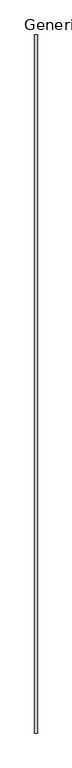
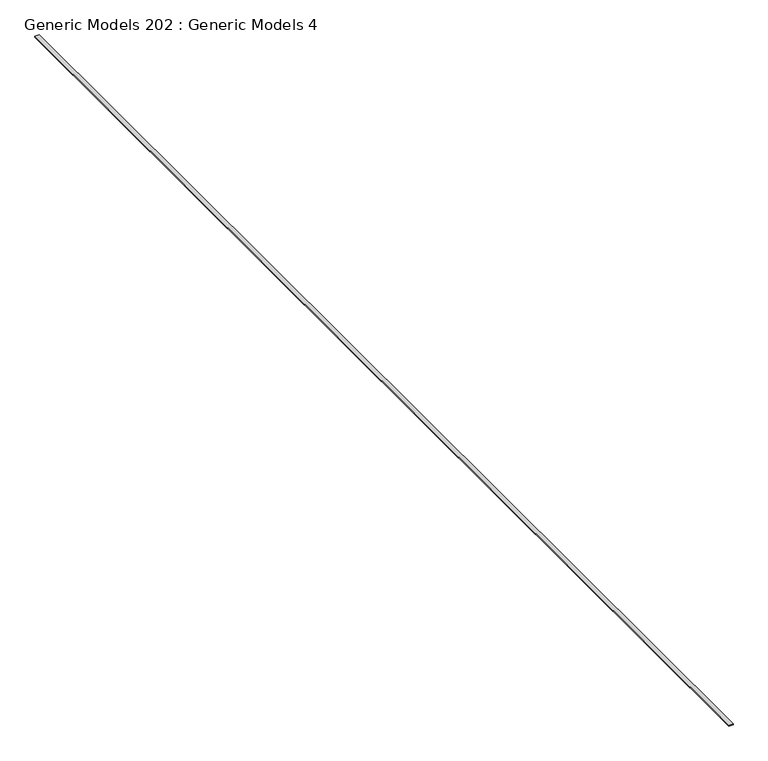
"""IFC4 building model written with IfcOpenShell, lengths in millimetres: proxy geometry, Generic Models 202 : Generic Models 4."""

from ifc_helpers import new_model, si_unit, frame, origin, place, context, project, spatial, polyline, outline, extrude, source, transform, mapped, element, save


def generic_models_202_generic_models_4_6e3a23b3(model_context):
    return source(origin(), model_context, "Body", "SweptSolid", [
        extrude(outline(polyline([(-8229.7736296, -1638.8730338), (-8280.5736296, -1638.8730338), (-8280.5736296, 11778.6769662), (-8229.7736296, 11778.6769662), (-8229.7736296, -1638.8730338)])), frame((0.0, 0.0, 127828.421), z_axis=(0.0, 0.0, 1.0), x_axis=(1.0, 0.0, 0.0)), (0.0, 0.0, 1.0), 12.263216),
    ])


if __name__ == "__main__":
    model = new_model("IFC4")
    model_context = context("Model", 3, world=origin())
    ifc_project = project(units=[si_unit("LENGTHUNIT", "METRE", prefix="MILLI")], contexts=[model_context])
    site = spatial("IfcSite", under=ifc_project)
    building = spatial("IfcBuilding", under=site)
    placement = place(None, origin())
    generic_models_202_generic_models_4_shape = generic_models_202_generic_models_4_6e3a23b3(model_context)
    element("IfcBuildingElementProxy", 1, Name="Generic Models 202 : Generic Models 4", ObjectType="Generic Models 202 : Generic Models 4", at=placement, inside=building, context=model_context, shape_type="MappedRepresentation", body=[
        mapped(generic_models_202_generic_models_4_shape, transform((0.0, 0.0, 0.0), x_axis=(1.0, 0.0, 0.0), y_axis=(0.0, 1.0, 0.0), z_axis=(0.0, 0.0, 1.0))),
    ])
    save(model, "model.ifc")

# Revit data of these elements
# Element 1 (IfcBuildingElementProxy, "Generic Models 202 : Generic Models 4")
#   Materials on its faces: "_3/4\" x 1 1/2\" STEEL FLAT STOCK (SCREWS COUNTERSUNK FROM BELOW)"
# Materials
#   "_3/4\" x 1 1/2\" STEEL FLAT STOCK (SCREWS COUNTERSUNK FROM BELOW)": class "Generic", colour RGB 233 233 233, transparency 0, Cost = 0
